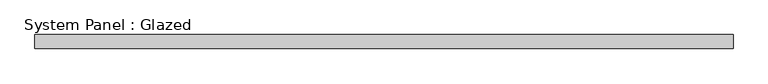
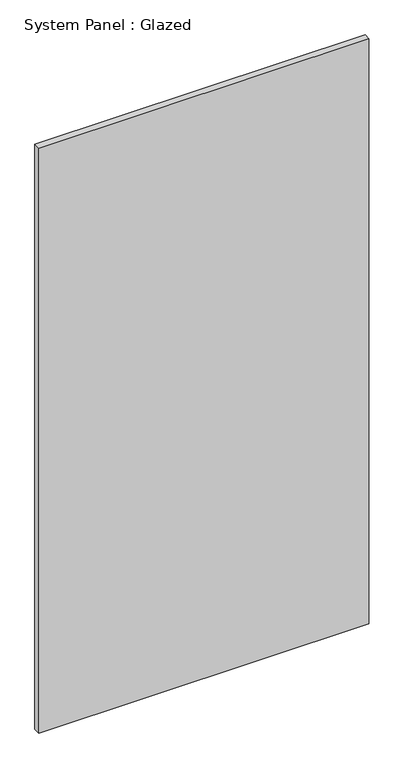
"""IFC4 building model written with IfcOpenShell, lengths in millimetres: plate geometry, System Panel : Glazed."""

import ifcopenshell
import ifcopenshell.guid

model = None  # the IFC model being written
_history = None  # IfcOwnerHistory: only IFC2X3 demands one
_inside = {}  # id of a spatial element -> (the spatial element, [elements in it])
_under = {}  # id of a project, library or spatial element -> (it, [spatial elements below it])
_declared = {}  # id of a project -> (the project, [libraries it declares])
_typed = {}  # id of a type object -> (the type object, [elements of that type])
_made_of = {}  # id of a material, layer set ... -> (it, [elements and type objects made of it])


def new_model(schema):
    """Start an empty IFC model of exactly this schema.

    Asked for "IFC4X3", IfcOpenShell would pick the latest addendum, in which some entities
    have other attributes; the version numbers below select the first issue.
    IFC2X3 requires an IfcOwnerHistory on every rooted entity: one is made here for all.
    """
    global model, _history
    if schema == "IFC4X3":
        model = ifcopenshell.file(schema_version=(4, 3, 0, 0))
    else:
        model = ifcopenshell.file(schema=schema)
    _inside.clear()
    _under.clear()
    _declared.clear()
    _typed.clear()
    _made_of.clear()
    _history = None
    if model.schema == "IFC2X3":
        org = make("IfcOrganization", Name="unknown")
        user = make(
            "IfcPersonAndOrganization",
            ThePerson=make("IfcPerson", FamilyName="unknown"),
            TheOrganization=org,
        )
        app = make(
            "IfcApplication",
            ApplicationDeveloper=org,
            Version="unknown",
            ApplicationFullName="unknown",
            ApplicationIdentifier="unknown",
        )
        _history = make(
            "IfcOwnerHistory",
            OwningUser=user,
            OwningApplication=app,
            ChangeAction="ADDED",
            CreationDate=0,
        )
    return model


def make(cls, **values):
    """One entity of the class cls with the attributes given. An attribute that is None is left unset."""
    return model.create_entity(
        cls, **{name: value for name, value in values.items() if value is not None}
    )


def rooted(cls, **values):
    """An entity with a GlobalId (a new one), such as an element, a storey or a relation."""
    return make(cls, GlobalId=ifcopenshell.guid.new(), OwnerHistory=_history, **values)


def si_unit(unit_type, name, prefix=None):
    """IfcSIUnit, for example si_unit("LENGTHUNIT", "METRE", prefix="MILLI")."""
    return make("IfcSIUnit", UnitType=unit_type, Prefix=prefix, Name=name)


def assignment(units):
    """IfcUnitAssignment: the units of a project."""
    return None if units is None else make("IfcUnitAssignment", Units=units)


def point(xyz):
    """IfcCartesianPoint."""
    return None if xyz is None else make("IfcCartesianPoint", Coordinates=xyz)


def direction(xyz):
    """IfcDirection."""
    return None if xyz is None else make("IfcDirection", DirectionRatios=xyz)


def frame(location, z_axis=None, x_axis=None):
    """IfcAxis2Placement3D, a coordinate frame: its origin and axes. An axis left out is left unset."""
    return make(
        "IfcAxis2Placement3D",
        Location=point(location),
        Axis=direction(z_axis),
        RefDirection=direction(x_axis),
    )


def origin():
    """The frame at (0, 0, 0) with its axes left unset."""
    return frame((0.0, 0.0, 0.0))


def origin_with_axes():
    """The frame at (0, 0, 0) with the z axis (0, 0, 1) and the x axis (1, 0, 0) written out."""
    return frame((0.0, 0.0, 0.0), z_axis=(0.0, 0.0, 1.0), x_axis=(1.0, 0.0, 0.0))


def place(relative_to, where):
    """IfcLocalPlacement: puts the frame where relative to a parent placement (None: the world)."""
    return make(
        "IfcLocalPlacement", PlacementRelTo=relative_to, RelativePlacement=where
    )


def context(
    kind, dimensions, precision=None, world=None, true_north=None, identifier=None
):
    """IfcGeometricRepresentationContext, for example the 3D "Model" context."""
    return make(
        "IfcGeometricRepresentationContext",
        ContextIdentifier=identifier,
        ContextType=kind,
        CoordinateSpaceDimension=dimensions,
        Precision=precision,
        WorldCoordinateSystem=world,
        TrueNorth=true_north,
    )


def project(units=None, contexts=None):
    """IfcProject with its units and contexts."""
    return rooted(
        "IfcProject",
        Name="project",
        RepresentationContexts=contexts,
        UnitsInContext=assignment(units),
    )


def spatial(cls, under=None, at=None, **own):
    """A site, building, storey or space (cls), placed at a placement, below another one or the project."""
    s = rooted(cls, ObjectPlacement=at, **own)
    if under is not None:
        _under.setdefault(under.id(), (under, []))[1].append(s)
    return s


def polyline(points):
    """IfcPolyline through the points."""
    return make("IfcPolyline", Points=[point(p) for p in points])


def outline(outer, holes=None, kind="AREA"):
    """IfcArbitraryClosedProfileDef: a profile drawn as a closed curve; with holes, ...WithVoids."""
    if holes is None:
        return make("IfcArbitraryClosedProfileDef", ProfileType=kind, OuterCurve=outer)
    return make(
        "IfcArbitraryProfileDefWithVoids",
        ProfileType=kind,
        OuterCurve=outer,
        InnerCurves=holes,
    )


def extrude(swept, where, along, depth):
    """IfcExtrudedAreaSolid: the profile swept, set in the frame where, extruded along a direction by depth."""
    return make(
        "IfcExtrudedAreaSolid",
        SweptArea=swept,
        Position=where,
        ExtrudedDirection=direction(along),
        Depth=depth,
    )


def shape(context_of_items, identifier, shape_type, items):
    """IfcShapeRepresentation: the items that make up one representation, for example the "Body"."""
    return make(
        "IfcShapeRepresentation",
        ContextOfItems=context_of_items,
        RepresentationIdentifier=identifier,
        RepresentationType=shape_type,
        Items=items,
    )


def source(mapping_origin, context_of_items, identifier, shape_type, items):
    """IfcRepresentationMap: a shape defined once, which mapped items show again and again."""
    return make(
        "IfcRepresentationMap",
        MappingOrigin=mapping_origin,
        MappedRepresentation=shape(context_of_items, identifier, shape_type, items),
    )


def transform(
    local_origin,
    x_axis=None,
    y_axis=None,
    z_axis=None,
    scale=None,
    scale2=None,
    scale3=None,
    uniform=True,
):
    """IfcCartesianTransformationOperator3D, or its non-uniform kind. x_axis, y_axis, z_axis: its Axis1, 2, 3."""
    if uniform:
        return make(
            "IfcCartesianTransformationOperator3D",
            Axis1=direction(x_axis),
            Axis2=direction(y_axis),
            LocalOrigin=point(local_origin),
            Scale=scale,
            Axis3=direction(z_axis),
        )
    return make(
        "IfcCartesianTransformationOperator3DnonUniform",
        Axis1=direction(x_axis),
        Axis2=direction(y_axis),
        LocalOrigin=point(local_origin),
        Scale=scale,
        Axis3=direction(z_axis),
        Scale2=scale2,
        Scale3=scale3,
    )


def mapped(mapping_source, mapping_target):
    """IfcMappedItem: shows the shape of a source again, moved by a transform."""
    return make(
        "IfcMappedItem", MappingSource=mapping_source, MappingTarget=mapping_target
    )


def made_of(thing, what):
    """Note that an element or type object is made of a material, layer set ...; save() writes the relation."""
    if what is not None:
        _made_of.setdefault(what.id(), (what, []))[1].append(thing)
    return thing


def element(
    cls,
    number,
    at=None,
    inside=None,
    cuts=None,
    type_object=None,
    material=None,
    context=None,
    identifier="Body",
    shape_type=None,
    held_by="IfcProductDefinitionShape",
    body=None,
    shapes=None,
    **own,
):
    """One element of the class cls, such as IfcWall. Its Tag is "e" and its number.

    at: its placement. inside: the storey or other place that contains it. cuts: it is an
    opening in that element (IfcRelVoidsElement). A single representation is given by context,
    identifier, shape_type and body (its items); several are given by shapes. held_by: the class
    of the entity that holds the representations. save() writes the other relations.
    """
    e = rooted(cls, Tag="e%d" % number, ObjectPlacement=at, **own)
    if body is not None:
        shapes = [shape(context, identifier, shape_type, body)]
    if shapes is not None:
        e.Representation = make(held_by, Representations=shapes)
    if inside is not None:
        _inside.setdefault(inside.id(), (inside, []))[1].append(e)
    if cuts is not None:
        rooted(
            "IfcRelVoidsElement", RelatingBuildingElement=cuts, RelatedOpeningElement=e
        )
    if type_object is not None:
        _typed.setdefault(type_object.id(), (type_object, []))[1].append(e)
    return made_of(e, material)


def aggregate(whole, parts):
    """IfcRelAggregates: a whole, such as a stair, and the parts it consists of."""
    return rooted("IfcRelAggregates", RelatingObject=whole, RelatedObjects=parts)


def save(model, path):
    """Write the relations noted so far, then the file.

    IfcRelAggregates (storeys below a building ...), IfcRelContainedInSpatialStructure (elements
    in a storey), IfcRelDefinesByType, IfcRelAssociatesMaterial and IfcRelDeclares: one each for
    every whole, place, type object, material and project.
    """
    for whole, parts in _under.values():
        aggregate(whole, parts)
    for where, things in _inside.values():
        rooted(
            "IfcRelContainedInSpatialStructure",
            RelatedElements=things,
            RelatingStructure=where,
        )
    for kind, things in _typed.values():
        rooted("IfcRelDefinesByType", RelatedObjects=things, RelatingType=kind)
    for what, things in _made_of.values():
        rooted("IfcRelAssociatesMaterial", RelatedObjects=things, RelatingMaterial=what)
    for by, libraries in _declared.values():
        rooted("IfcRelDeclares", RelatingContext=by, RelatedDefinitions=libraries)
    model.write(path)


def system_panel_glazed_6c662813(model_context):
    return source(origin(), model_context, "Body", "SweptSolid", [
        extrude(outline(polyline([(620.5541356, 24.5), (-620.5541356, 24.5), (-620.5541356, 49.5), (620.5541356, 49.5), (620.5541356, 24.5)])), origin_with_axes(), (0.0, 0.0, 1.0), 2325.0),
    ])


if __name__ == "__main__":
    model = new_model("IFC4")
    model_context = context("Model", 3, world=origin())
    ifc_project = project(units=[si_unit("LENGTHUNIT", "METRE", prefix="MILLI")], contexts=[model_context])
    site = spatial("IfcSite", under=ifc_project)
    building = spatial("IfcBuilding", under=site)
    placement = place(None, origin())
    system_panel_glazed_shape = system_panel_glazed_6c662813(model_context)
    element("IfcPlate", 1, ObjectType="System Panel : Glazed", at=placement, inside=building, context=model_context, shape_type="MappedRepresentation", body=[
        mapped(system_panel_glazed_shape, transform((0.0, 0.0, 0.0), x_axis=(1.0, 0.0, 0.0), y_axis=(0.0, 1.0, 0.0), z_axis=(0.0, 0.0, 1.0))),
    ])
    save(model, "model.ifc")

# Revit data of these elements
# Type "System Panel : Glazed"
#   Construction Type Id = "GSP4R"
#   Analytic Construction = "1/8 in Pilkington single glazing"
#   Visual Light Transmittance = 0.9
#   Solar Heat Gain Coefficient = 0.86
#   Heat Transfer Coefficient (U) = 6.7069 W/(m²·K)
#   Define Thermal Properties by = 1
# Element 1 (IfcPlate, "System Panel : Glazed")
#   Materials on its faces: "Glass"
# Materials
#   "Glass": class "Glass", colour RGB 0 128 192, transparency 0.9, Description = "Soda Lime Glass", Cost = 0
